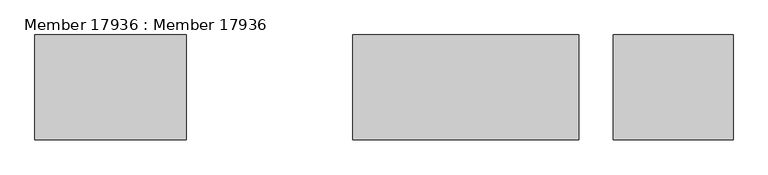
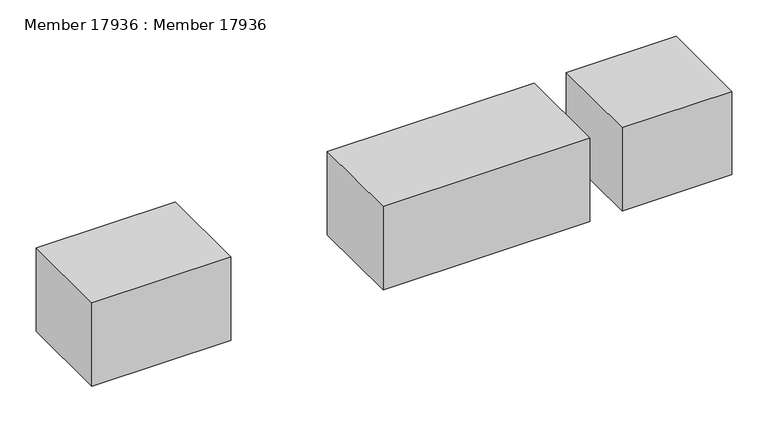
"""IFC4 building model written with IfcOpenShell, lengths in millimetres: proxy geometry, Member 17936 : Member 17936."""

from ifc_helpers import new_model, si_unit, frame, origin, place, context, project, spatial, polyline, outline, extrude, source, transform, mapped, element, save


def member_17936_member_17936_6a1f500c(model_context):
    return source(origin(), model_context, "Body", "SweptSolid", [
        extrude(outline(polyline([(8058.8506189, -1900.3491938), (7730.7851931, -1900.3491938), (7730.7851931, -1747.9491938), (8058.8506189, -1747.9491938), (8058.8506189, -1900.3491938)])), frame((0.0, 0.0, 39572.9453124), z_axis=(0.0, 0.0, 1.0), x_axis=(1.0, 0.0, 0.0)), (0.0, 0.0, 1.0), 139.7006876),
        extrude(outline(polyline([(7489.4851931, -1900.3491938), (7269.3762048, -1900.3491938), (7269.3762048, -1747.9491938), (7489.4851931, -1747.9491938), (7489.4851931, -1900.3491938)])), frame((0.0, 0.0, 39572.946), z_axis=(0.0, 0.0, 1.0), x_axis=(1.0, 0.0, 0.0)), (0.0, 0.0, 1.0), 139.7),
        extrude(outline(polyline([(8283.3477835, -1900.3491938), (8109.6506189, -1900.3491938), (8109.6506189, -1747.9491938), (8283.3477835, -1747.9491938), (8283.3477835, -1900.3491938)])), frame((0.0, 0.0, 39572.946), z_axis=(0.0, 0.0, 1.0), x_axis=(1.0, 0.0, 0.0)), (0.0, 0.0, 1.0), 139.7),
    ])


if __name__ == "__main__":
    model = new_model("IFC4")
    model_context = context("Model", 3, world=origin())
    ifc_project = project(units=[si_unit("LENGTHUNIT", "METRE", prefix="MILLI")], contexts=[model_context])
    site = spatial("IfcSite", under=ifc_project)
    building = spatial("IfcBuilding", under=site)
    placement = place(None, origin())
    member_17936_member_17936_shape = member_17936_member_17936_6a1f500c(model_context)
    element("IfcBuildingElementProxy", 1, Name="Member 17936 : Member 17936", ObjectType="Member 17936 : Member 17936", at=placement, inside=building, context=model_context, shape_type="MappedRepresentation", body=[
        mapped(member_17936_member_17936_shape, transform((0.0, 0.0, 0.0), x_axis=(1.0, 0.0, 0.0), y_axis=(0.0, 1.0, 0.0), z_axis=(0.0, 0.0, 1.0))),
    ])
    save(model, "model.ifc")

# Revit data of these elements
# Type "Member 17936 : Member 17936"
#   NameOverride = "Member"
# Element 1 (IfcBuildingElementProxy, "Member 17936 : Member 17936")
#   Materials on its faces: "WOOD FRAMING (SEE STRUCT DWGS)"
# Materials
#   "WOOD FRAMING (SEE STRUCT DWGS)": class "Unassigned", colour RGB 224 188 168, transparency 0, Cost = 0
